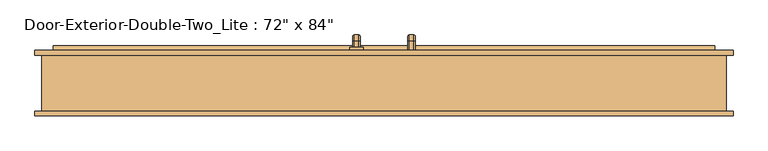
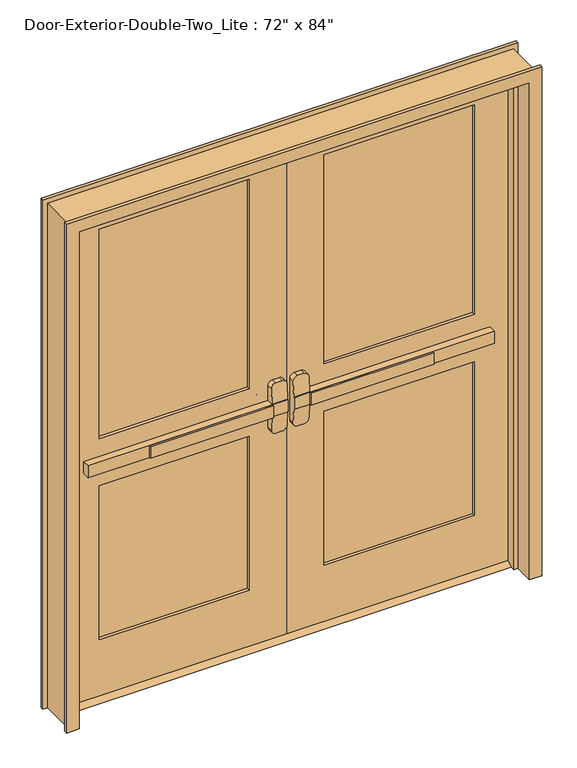
"""IFC4 building model written with IfcOpenShell, lengths in millimetres: door geometry."""

from ifc_helpers import new_model, si_unit, point, frame, frame_2d, origin, place, context, project, spatial, polyline, circle_curve, ellipse_curve, trimmed, segment, composite_curve, outline, extrude, faceted_brep, source, transform, mapped, element, save
from ifc_brep_helpers import plane_surface, cylinder_surface, revolved_surface, advanced_brep


def door_a6d348c0(model_context):
    return source(origin(), model_context, "Body", "SolidModel", [
        extrude(outline(polyline([(-575.7333333, 1.5875), (-575.7333333, 7.9375), (-76.2, 7.9375), (-76.2, 1.5875), (-575.7333333, 1.5875)])), frame((0.0, 0.0, 990.6), z_axis=(0.0, 0.0, 1.0), x_axis=(1.0, 0.0, 0.0)), (0.0, 0.0, 1.0), 50.8),
        advanced_brep(
        [(-12.7, 7.9375, 1041.4), (-76.2, 7.9375, 1041.4), (-825.5, 7.9375, 1041.4), (-825.5, 7.9375, 990.6), (-76.2, 7.9375, 990.6), (-12.7, 7.9375, 990.6), (-825.5, 39.6875, 1041.4), (-76.2, 39.6875, 1041.4), (-76.2, 39.6875, 1104.9), (-57.15, 39.6875, 1123.95), (-31.75, 39.6875, 1123.95), (-12.7, 39.6875, 1104.9), (-12.7, 39.6875, 927.1), (-31.75, 39.6875, 908.05), (-57.15, 39.6875, 908.05), (-76.2, 39.6875, 927.1), (-76.2, 39.6875, 990.6), (-825.5, 39.6875, 990.6), (-12.7, 11.1127467, 1041.4), (-76.2, 11.1127467, 1041.4), (-12.7, 11.1127467, 990.6), (-12.7, 16.1229269, 927.1), (-12.7, 16.1229269, 1104.9), (-76.2, 11.1127467, 990.6), (-76.2, 16.1229269, 1104.9), (-76.2, 16.1229269, 927.1), (-57.15, 17.625981, 1123.95), (-31.75, 17.625981, 1123.95), (-31.75, 17.625981, 908.05), (-57.15, 17.625981, 908.05)],
        [
            (0, 1),
            (1, 2),
            (2, 3),
            (3, 4),
            (4, 5),
            (5, 0),
            (6, 7),
            (7, 8),
            (8, 9, circle_curve(frame((-57.15, 39.6875, 1104.9), z_axis=(0.0, 1.0, 0.0), x_axis=(-1.0, 0.0, 0.0)), 19.05)),
            (9, 10),
            (10, 11, circle_curve(frame((-31.75, 39.6875, 1104.9), z_axis=(0.0, 1.0, 0.0), x_axis=(-1.0, 0.0, 0.0)), 19.05)),
            (11, 12),
            (12, 13, circle_curve(frame((-31.75, 39.6875, 927.1), z_axis=(0.0, 1.0, 0.0), x_axis=(-1.0, 0.0, 0.0)), 19.05)),
            (13, 14),
            (14, 15, circle_curve(frame((-57.15, 39.6875, 927.1), z_axis=(0.0, 1.0, 0.0), x_axis=(-1.0, 0.0, 0.0)), 19.05)),
            (15, 16),
            (16, 17),
            (17, 6),
            (0, 18),
            (18, 19),
            (19, 7),
            (6, 2),
            (5, 20),
            (20, 21),
            (21, 12),
            (11, 22),
            (22, 18),
            (16, 23),
            (23, 20),
            (3, 17),
            (19, 24),
            (24, 8),
            (15, 25),
            (25, 23),
            (9, 26),
            (26, 27),
            (27, 10),
            (13, 28),
            (28, 29),
            (29, 14),
            (29, 25, ellipse_curve(frame((-57.15, 16.1229269, 927.1), z_axis=(0.0, 0.9969018152893365, 0.07865602756830282), x_axis=(0.0, -0.07865602756830208, 0.9969018152893365)), 19.1092038, 19.05)),
            (24, 26, ellipse_curve(frame((-57.15, 16.1229269, 1104.9), z_axis=(0.0, 0.9969018152893376, -0.07865602756828934), x_axis=(0.0, -0.078656027568288, -0.9969018152893377)), 19.1092038, 19.05)),
            (27, 22, ellipse_curve(frame((-31.75, 16.1229269, 1104.9), z_axis=(0.0, 0.9969018152893376, -0.07865602756828934), x_axis=(0.0, -0.078656027568288, -0.9969018152893377)), 19.1092038, 19.05)),
            (21, 28, ellipse_curve(frame((-31.75, 16.1229269, 927.1), z_axis=(0.0, 0.9969018152893365, 0.07865602756830282), x_axis=(0.0, -0.07865602756830208, 0.9969018152893365)), 19.1092038, 19.05)),
        ],
        [
            plane_surface(frame((-12.7, 7.9375, 1041.4), z_axis=(0.0, -1.0, 0.0), x_axis=(1.0, 0.0, 0.0))),
            plane_surface(frame((-12.7, 39.6875, 1041.4), z_axis=(0.0, 1.0, 0.0), x_axis=(-1.0, 0.0, 0.0))),
            plane_surface(frame((-825.5, 7.9375, 1041.4), z_axis=(0.0, 0.0, 1.0), x_axis=(0.0, 1.0, 0.0))),
            plane_surface(frame((-12.7, 7.9375, 1041.4), z_axis=(1.0, 0.0, 0.0), x_axis=(0.0, 1.0, 0.0))),
            plane_surface(frame((-12.7, 7.9375, 990.6), z_axis=(0.0, 0.0, -1.0), x_axis=(0.0, 1.0, 0.0))),
            plane_surface(frame((-825.5, 7.9375, 990.6), z_axis=(-1.0, 0.0, 0.0), x_axis=(0.0, 1.0, 0.0))),
            plane_surface(frame((-76.2, 11.1127467, 927.1), z_axis=(-1.0, 0.0, 0.0), x_axis=(0.0, 1.0, 0.0))),
            plane_surface(frame((-57.15, 11.1127467, 1123.95), z_axis=(0.0, 0.0, 1.0), x_axis=(0.0, 1.0, 0.0))),
            plane_surface(frame((-31.75, 11.1127467, 908.05), z_axis=(0.0, 0.0, -1.0), x_axis=(0.0, 1.0, 0.0))),
            cylinder_surface(frame((-57.15, 39.6875, 927.1), z_axis=(0.0, -1.0, 0.0), x_axis=(-1.0, 0.0, 0.0)), 19.05),
            cylinder_surface(frame((-57.15, 39.6875, 1104.9), z_axis=(0.0, -1.0, 0.0), x_axis=(-1.0, 0.0, 0.0)), 19.05),
            cylinder_surface(frame((-31.75, 39.6875, 1104.9), z_axis=(0.0, -1.0, 0.0), x_axis=(-1.0, 0.0, 0.0)), 19.05),
            cylinder_surface(frame((-31.75, 39.6875, 927.1), z_axis=(0.0, -1.0, 0.0), x_axis=(-1.0, 0.0, 0.0)), 19.05),
            plane_surface(frame((-76.2, 11.1127467, 1041.4), z_axis=(0.0, -0.9969018152893376, 0.07865602756828934), x_axis=(1.0, 0.0, 0.0))),
            plane_surface(frame((-76.2, 17.625981, 908.05), z_axis=(0.0, -0.9969018152893365, -0.07865602756830282), x_axis=(1.0, 0.0, 0.0))),
        ],
        [
            (0, [[1, 2, 3, 4, 5, 6]]),
            (1, [[7, 8, 9, 10, 11, 12, 13, 14, 15, 16, 17, 18]]),
            (2, [[-2, -1, 19, 20, 21, -7, 22]]),
            (3, [[23, 24, 25, -12, 26, 27, -19, -6]]),
            (4, [[-17, 28, 29, -23, -5, -4, 30]]),
            (5, [[-22, -18, -30, -3]]),
            (6, [[-21, 31, 32, -8]]),
            (6, [[33, 34, -28, -16]]),
            (7, [[35, 36, 37, -10]]),
            (8, [[38, 39, 40, -14]]),
            (9, [[-40, 41, -33, -15]]),
            (10, [[-32, 42, -35, -9]]),
            (11, [[-37, 43, -26, -11]]),
            (12, [[-25, 44, -38, -13]]),
            (13, [[-27, -43, -36, -42, -31, -20]]),
            (14, [[-29, -34, -41, -39, -44, -24]]),
        ],
    ),
        extrude(outline(polyline([(84.1375, 12.7), (109.5375, 0.0), (14.2875, 0.0), (39.6875, 12.7), (84.1375, 12.7)])), frame((-914.4, 0.0, 0.0), z_axis=(1.0, 0.0, 0.0), x_axis=(0.0, 1.0, 0.0)), (0.0, 0.0, 1.0), 1828.8),
        extrude(outline(polyline([(575.7333333, 1.5875), (76.2, 1.5875), (76.2, 7.9375), (575.7333333, 7.9375), (575.7333333, 1.5875)])), frame((0.0, 0.0, 990.6), z_axis=(0.0, 0.0, 1.0), x_axis=(1.0, 0.0, 0.0)), (0.0, 0.0, 1.0), 50.8),
        advanced_brep(
        [(12.7, 7.9375, 1041.4), (12.7, 7.9375, 990.6), (76.2, 7.9375, 990.6), (825.5, 7.9375, 990.6), (825.5, 7.9375, 1041.4), (76.2, 7.9375, 1041.4), (825.5, 39.6875, 1041.4), (825.5, 39.6875, 990.6), (76.2, 39.6875, 990.6), (76.2, 39.6875, 927.1), (57.15, 39.6875, 908.05), (31.75, 39.6875, 908.05), (12.7, 39.6875, 927.1), (12.7, 39.6875, 1104.9), (31.75, 39.6875, 1123.95), (57.15, 39.6875, 1123.95), (76.2, 39.6875, 1104.9), (76.2, 39.6875, 1041.4), (76.2, 11.1127467, 1041.4), (12.7, 11.1127467, 1041.4), (12.7, 16.1229269, 1104.9), (12.7, 16.1229269, 927.1), (12.7, 11.1127467, 990.6), (76.2, 11.1127467, 990.6), (76.2, 16.1229269, 927.1), (76.2, 16.1229269, 1104.9), (31.75, 17.625981, 1123.95), (57.15, 17.625981, 1123.95), (57.15, 17.625981, 908.05), (31.75, 17.625981, 908.05)],
        [
            (0, 1),
            (1, 2),
            (2, 3),
            (3, 4),
            (4, 5),
            (5, 0),
            (6, 7),
            (7, 8),
            (8, 9),
            (9, 10, circle_curve(frame((57.15, 39.6875, 927.1), z_axis=(0.0, 1.0, 0.0), x_axis=(1.0, 0.0, 0.0)), 19.05)),
            (10, 11),
            (11, 12, circle_curve(frame((31.75, 39.6875, 927.1), z_axis=(0.0, 1.0, 0.0), x_axis=(1.0, 0.0, 0.0)), 19.05)),
            (12, 13),
            (13, 14, circle_curve(frame((31.75, 39.6875, 1104.9), z_axis=(0.0, 1.0, 0.0), x_axis=(1.0, 0.0, 0.0)), 19.05)),
            (14, 15),
            (15, 16, circle_curve(frame((57.15, 39.6875, 1104.9), z_axis=(0.0, 1.0, 0.0), x_axis=(1.0, 0.0, 0.0)), 19.05)),
            (16, 17),
            (17, 6),
            (4, 6),
            (17, 18),
            (18, 19),
            (19, 0),
            (19, 20),
            (20, 13),
            (12, 21),
            (21, 22),
            (22, 1),
            (7, 3),
            (22, 23),
            (23, 8),
            (23, 24),
            (24, 9),
            (16, 25),
            (25, 18),
            (14, 26),
            (26, 27),
            (27, 15),
            (10, 28),
            (28, 29),
            (29, 11),
            (24, 28, ellipse_curve(frame((57.15, 16.1229269, 927.1), z_axis=(0.0, 0.9969018152893365, 0.07865602756830282), x_axis=(0.0, -0.07865602756830208, 0.9969018152893365)), 19.1092038, 19.05)),
            (27, 25, ellipse_curve(frame((57.15, 16.1229269, 1104.9), z_axis=(0.0, 0.9969018152893376, -0.07865602756828934), x_axis=(0.0, -0.078656027568288, -0.9969018152893377)), 19.1092038, 19.05)),
            (20, 26, ellipse_curve(frame((31.75, 16.1229269, 1104.9), z_axis=(0.0, 0.9969018152893376, -0.07865602756828934), x_axis=(0.0, -0.078656027568288, -0.9969018152893377)), 19.1092038, 19.05)),
            (29, 21, ellipse_curve(frame((31.75, 16.1229269, 927.1), z_axis=(0.0, 0.9969018152893365, 0.07865602756830282), x_axis=(0.0, -0.07865602756830208, 0.9969018152893365)), 19.1092038, 19.05)),
        ],
        [
            plane_surface(frame((12.7, 7.9375, 1041.4), z_axis=(0.0, -1.0, 0.0), x_axis=(-1.0, 0.0, 0.0))),
            plane_surface(frame((12.7, 39.6875, 1041.4), z_axis=(0.0, 1.0, 0.0), x_axis=(1.0, 0.0, 0.0))),
            plane_surface(frame((825.5, 7.9375, 1041.4), z_axis=(0.0, 0.0, 1.0), x_axis=(0.0, 1.0, 0.0))),
            plane_surface(frame((12.7, 7.9375, 1041.4), z_axis=(-1.0, 0.0, 0.0), x_axis=(0.0, 1.0, 0.0))),
            plane_surface(frame((12.7, 7.9375, 990.6), z_axis=(0.0, 0.0, -1.0), x_axis=(0.0, 1.0, 0.0))),
            plane_surface(frame((825.5, 7.9375, 990.6), z_axis=(1.0, 0.0, 0.0), x_axis=(0.0, 1.0, 0.0))),
            plane_surface(frame((76.2, 11.1127467, 927.1), z_axis=(1.0, 0.0, 0.0), x_axis=(0.0, 1.0, 0.0))),
            plane_surface(frame((57.15, 11.1127467, 1123.95), z_axis=(0.0, 0.0, 1.0), x_axis=(0.0, 1.0, 0.0))),
            plane_surface(frame((31.75, 11.1127467, 908.05), z_axis=(0.0, 0.0, -1.0), x_axis=(0.0, 1.0, 0.0))),
            cylinder_surface(frame((57.15, 39.6875, 927.1), z_axis=(0.0, -1.0, 0.0), x_axis=(1.0, 0.0, 0.0)), 19.05),
            cylinder_surface(frame((57.15, 39.6875, 1104.9), z_axis=(0.0, -1.0, 0.0), x_axis=(1.0, 0.0, 0.0)), 19.05),
            cylinder_surface(frame((31.75, 39.6875, 1104.9), z_axis=(0.0, -1.0, 0.0), x_axis=(1.0, 0.0, 0.0)), 19.05),
            cylinder_surface(frame((31.75, 39.6875, 927.1), z_axis=(0.0, -1.0, 0.0), x_axis=(1.0, 0.0, 0.0)), 19.05),
            plane_surface(frame((76.2, 11.1127467, 1041.4), z_axis=(0.0, -0.9969018152893376, 0.07865602756828934), x_axis=(-1.0, 0.0, 0.0))),
            plane_surface(frame((76.2, 17.625981, 908.05), z_axis=(0.0, -0.9969018152893365, -0.07865602756830282), x_axis=(-1.0, 0.0, 0.0))),
        ],
        [
            (0, [[1, 2, 3, 4, 5, 6]]),
            (1, [[7, 8, 9, 10, 11, 12, 13, 14, 15, 16, 17, 18]]),
            (2, [[19, -18, 20, 21, 22, -6, -5]]),
            (3, [[-1, -22, 23, 24, -13, 25, 26, 27]]),
            (4, [[28, -3, -2, -27, 29, 30, -8]]),
            (5, [[-4, -28, -7, -19]]),
            (6, [[-9, -30, 31, 32]]),
            (6, [[-17, 33, 34, -20]]),
            (7, [[-15, 35, 36, 37]]),
            (8, [[-11, 38, 39, 40]]),
            (9, [[-10, -32, 41, -38]]),
            (10, [[-16, -37, 42, -33]]),
            (11, [[-14, -24, 43, -35]]),
            (12, [[-12, -40, 44, -25]]),
            (13, [[-21, -34, -42, -36, -43, -23]]),
            (14, [[-26, -44, -39, -41, -31, -29]]),
        ],
    ),
        advanced_brep(
        [(66.2, 96.8375, 1017.190625), (66.2, 96.8375, 1014.809375), (69.771875, 96.8375, 1011.2375), (82.6284594, 96.8375, 1011.2375), (86.2, 96.8375, 1014.8090406), (86.2, 96.8375, 1017.190625), (82.628125, 96.8375, 1020.7625), (69.771875, 96.8375, 1020.7625), (66.2, 96.8375, 887.809375), (69.771875, 96.8375, 884.2375), (82.628125, 96.8375, 884.2375), (86.2, 96.8375, 887.809375), (86.2, 96.8375, 890.1909594), (82.6284594, 96.8375, 893.7625), (69.771875, 96.8375, 893.7625), (66.2, 96.8375, 890.190625), (66.2, 122.2375, 1017.190625), (66.2, 136.128125, 1003.3), (66.2, 136.128125, 901.7), (66.2, 122.2375, 887.809375), (66.2, 122.2375, 890.190625), (66.2, 133.746875, 901.7), (66.2, 133.746875, 1003.3), (66.2, 122.2375, 1014.809375), (69.771875, 122.2375, 1011.2375), (82.6284594, 122.2375, 1011.2375), (86.2, 122.2375, 1014.8090406), (86.2, 133.7465406, 1003.3), (86.2, 133.7465406, 901.7), (86.2, 122.2375, 890.1909594), (86.2, 122.2375, 887.809375), (86.2, 136.128125, 901.7), (86.2, 136.128125, 1003.3), (86.2, 122.2375, 1017.190625), (82.628125, 122.2375, 1020.7625), (69.771875, 122.2375, 1020.7625), (69.771875, 130.175, 1003.3), (82.6284594, 130.175, 1003.3), (82.628125, 139.7, 1003.3), (69.771875, 139.7, 1003.3), (69.771875, 130.175, 901.7), (82.6284594, 130.175, 901.7), (82.628125, 139.7, 901.7), (69.771875, 139.7, 901.7), (69.771875, 122.2375, 893.7625), (82.6284594, 122.2375, 893.7625), (82.628125, 122.2375, 884.2375), (69.771875, 122.2375, 884.2375)],
        [
            (0, 1),
            (1, 2, circle_curve(frame((69.771875, 96.8375, 1014.809375), z_axis=(0.0, -1.0, 0.0), x_axis=(0.0, 0.0, 1.0)), 3.571875)),
            (2, 3),
            (3, 4, circle_curve(frame((82.6284594, 96.8375, 1014.8090406), z_axis=(0.0, -1.0, 0.0), x_axis=(0.0, 0.0, 1.0)), 3.5715406)),
            (4, 5),
            (5, 6, circle_curve(frame((82.628125, 96.8375, 1017.190625), z_axis=(0.0, -1.0, 0.0), x_axis=(0.0, 0.0, 1.0)), 3.571875)),
            (6, 7),
            (7, 0, circle_curve(frame((69.771875, 96.8375, 1017.190625), z_axis=(0.0, -1.0, 0.0), x_axis=(0.0, 0.0, 1.0)), 3.571875)),
            (8, 9, circle_curve(frame((69.771875, 96.8375, 887.809375), z_axis=(0.0, -1.0, 0.0), x_axis=(0.0, 0.0, -1.0)), 3.571875)),
            (9, 10),
            (10, 11, circle_curve(frame((82.628125, 96.8375, 887.809375), z_axis=(0.0, -1.0, 0.0), x_axis=(0.0, 0.0, -1.0)), 3.571875)),
            (11, 12),
            (12, 13, circle_curve(frame((82.6284594, 96.8375, 890.1909594), z_axis=(0.0, -1.0, 0.0), x_axis=(0.0, 0.0, -1.0)), 3.5715406)),
            (13, 14),
            (14, 15, circle_curve(frame((69.771875, 96.8375, 890.190625), z_axis=(0.0, -1.0, 0.0), x_axis=(0.0, 0.0, -1.0)), 3.571875)),
            (15, 8),
            (0, 16),
            (16, 17, circle_curve(frame((66.2, 122.2375, 1003.3), z_axis=(-1.0, 0.0, 0.0), x_axis=(0.0, 0.0, 1.0)), 13.890625)),
            (17, 18),
            (18, 19, circle_curve(frame((66.2, 122.2375, 901.7), z_axis=(-1.0, 0.0, 0.0), x_axis=(0.0, 1.0, 0.0)), 13.890625)),
            (19, 8),
            (15, 20),
            (20, 21, circle_curve(frame((66.2, 122.2375, 901.7), z_axis=(1.0, 0.0, 0.0), x_axis=(0.0, 1.0, 0.0)), 11.509375)),
            (21, 22),
            (22, 23, circle_curve(frame((66.2, 122.2375, 1003.3), z_axis=(1.0, 0.0, 0.0), x_axis=(0.0, 0.0, 1.0)), 11.509375)),
            (23, 1),
            (23, 24, circle_curve(frame((69.771875, 122.2375, 1014.809375), z_axis=(0.0, -1.0, 0.0), x_axis=(0.0, 0.0, 1.0)), 3.571875)),
            (24, 2),
            (24, 25),
            (25, 3),
            (25, 26, circle_curve(frame((82.6284594, 122.2375, 1014.8090406), z_axis=(0.0, -1.0, 0.0), x_axis=(0.0, 0.0, 1.0)), 3.5715406)),
            (26, 4),
            (26, 27, circle_curve(frame((86.2, 122.2375, 1003.3), z_axis=(-1.0, 0.0, 0.0), x_axis=(0.0, 0.0, 1.0)), 11.5090406)),
            (27, 28),
            (28, 29, circle_curve(frame((86.2, 122.2375, 901.7), z_axis=(-1.0, 0.0, 0.0), x_axis=(0.0, 1.0, 0.0)), 11.5090406)),
            (29, 12),
            (11, 30),
            (30, 31, circle_curve(frame((86.2, 122.2375, 901.7), z_axis=(1.0, 0.0, 0.0), x_axis=(0.0, 1.0, 0.0)), 13.890625)),
            (31, 32),
            (32, 33, circle_curve(frame((86.2, 122.2375, 1003.3), z_axis=(1.0, 0.0, 0.0), x_axis=(0.0, 0.0, 1.0)), 13.890625)),
            (33, 5),
            (33, 34, circle_curve(frame((82.628125, 122.2375, 1017.190625), z_axis=(0.0, -1.0, 0.0), x_axis=(0.0, 0.0, 1.0)), 3.571875)),
            (34, 6),
            (34, 35),
            (35, 7),
            (35, 16, circle_curve(frame((69.771875, 122.2375, 1017.190625), z_axis=(0.0, -1.0, 0.0), x_axis=(0.0, 0.0, 1.0)), 3.571875)),
            (36, 24, circle_curve(frame((69.771875, 122.2375, 1003.3), z_axis=(1.0, 0.0, 0.0), x_axis=(0.0, 0.0, 1.0)), 7.9375)),
            (22, 36, circle_curve(frame((69.771875, 133.746875, 1003.3), z_axis=(0.0, 0.0, 1.0), x_axis=(0.0, 1.0, 0.0)), 3.571875)),
            (37, 25, circle_curve(frame((82.6284594, 122.2375, 1003.3), z_axis=(1.0, 0.0, 0.0), x_axis=(0.0, 0.0, 1.0)), 7.9375)),
            (36, 37),
            (37, 27, circle_curve(frame((82.6284594, 133.7465406, 1003.3), z_axis=(0.0, 0.0, 1.0), x_axis=(0.0, 1.0, 0.0)), 3.5715406)),
            (38, 34, circle_curve(frame((82.628125, 122.2375, 1003.3), z_axis=(1.0, 0.0, 0.0), x_axis=(0.0, 0.0, 1.0)), 17.4625)),
            (32, 38, circle_curve(frame((82.628125, 136.128125, 1003.3), z_axis=(0.0, 0.0, 1.0), x_axis=(0.0, 1.0, 0.0)), 3.571875)),
            (39, 35, circle_curve(frame((69.771875, 122.2375, 1003.3), z_axis=(1.0, 0.0, 0.0), x_axis=(0.0, 0.0, 1.0)), 17.4625)),
            (38, 39),
            (39, 17, circle_curve(frame((69.771875, 136.128125, 1003.3), z_axis=(0.0, 0.0, 1.0), x_axis=(0.0, 1.0, 0.0)), 3.571875)),
            (21, 40, circle_curve(frame((69.771875, 133.746875, 901.7), z_axis=(0.0, 0.0, 1.0), x_axis=(0.0, 1.0, 0.0)), 3.571875)),
            (40, 36),
            (40, 41),
            (41, 37),
            (41, 28, circle_curve(frame((82.6284594, 133.7465406, 901.7), z_axis=(0.0, 0.0, 1.0), x_axis=(0.0, 1.0, 0.0)), 3.5715406)),
            (31, 42, circle_curve(frame((82.628125, 136.128125, 901.7), z_axis=(0.0, 0.0, 1.0), x_axis=(0.0, 1.0, 0.0)), 3.571875)),
            (42, 38),
            (42, 43),
            (43, 39),
            (43, 18, circle_curve(frame((69.771875, 136.128125, 901.7), z_axis=(0.0, 0.0, 1.0), x_axis=(0.0, 1.0, 0.0)), 3.571875)),
            (44, 40, circle_curve(frame((69.771875, 122.2375, 901.7), z_axis=(1.0, 0.0, 0.0), x_axis=(0.0, 1.0, 0.0)), 7.9375)),
            (20, 44, circle_curve(frame((69.771875, 122.2375, 890.190625), z_axis=(0.0, 1.0, 0.0), x_axis=(0.0, 0.0, -1.0)), 3.571875)),
            (45, 41, circle_curve(frame((82.6284594, 122.2375, 901.7), z_axis=(1.0, 0.0, 0.0), x_axis=(0.0, 1.0, 0.0)), 7.9375)),
            (44, 45),
            (45, 29, circle_curve(frame((82.6284594, 122.2375, 890.1909594), z_axis=(0.0, 1.0, 0.0), x_axis=(0.0, 0.0, -1.0)), 3.5715406)),
            (46, 42, circle_curve(frame((82.628125, 122.2375, 901.7), z_axis=(1.0, 0.0, 0.0), x_axis=(0.0, 1.0, 0.0)), 17.4625)),
            (30, 46, circle_curve(frame((82.628125, 122.2375, 887.809375), z_axis=(0.0, 1.0, 0.0), x_axis=(0.0, 0.0, -1.0)), 3.571875)),
            (47, 43, circle_curve(frame((69.771875, 122.2375, 901.7), z_axis=(1.0, 0.0, 0.0), x_axis=(0.0, 1.0, 0.0)), 17.4625)),
            (46, 47),
            (47, 19, circle_curve(frame((69.771875, 122.2375, 887.809375), z_axis=(0.0, 1.0, 0.0), x_axis=(0.0, 0.0, -1.0)), 3.571875)),
            (14, 44),
            (13, 45),
            (10, 46),
            (9, 47),
        ],
        [
            plane_surface(frame((76.2, 96.8375, 1016.0), z_axis=(0.0, -1.0, 0.0), x_axis=(1.0, 0.0, 0.0))),
            plane_surface(frame((76.2, 96.8375, 889.0), z_axis=(0.0, -1.0, 0.0), x_axis=(1.0, 0.0, 0.0))),
            plane_surface(frame((66.2, 96.8375, 1017.190625), z_axis=(-1.0, 0.0, 0.0), x_axis=(0.0, 1.0, 0.0))),
            cylinder_surface(frame((69.771875, 96.8375, 1014.809375), z_axis=(0.0, -1.0, 0.0), x_axis=(0.0, 0.0, 1.0)), 3.571875),
            plane_surface(frame((69.771875, 96.8375, 1011.2375), z_axis=(0.0, 0.0, -1.0), x_axis=(0.0, 1.0, 0.0))),
            cylinder_surface(frame((82.6284594, 96.8375, 1014.8090406), z_axis=(0.0, -1.0, 0.0), x_axis=(0.0, 0.0, 1.0)), 3.5715406),
            plane_surface(frame((86.2, 96.8375, 1014.8090406), z_axis=(1.0, 0.0, 0.0), x_axis=(0.0, 1.0, 0.0))),
            cylinder_surface(frame((82.628125, 96.8375, 1017.190625), z_axis=(0.0, -1.0, 0.0), x_axis=(0.0, 0.0, 1.0)), 3.571875),
            plane_surface(frame((82.628125, 96.8375, 1020.7625), z_axis=(0.0, 0.0, 1.0), x_axis=(0.0, 1.0, 0.0))),
            cylinder_surface(frame((69.771875, 96.8375, 1017.190625), z_axis=(0.0, -1.0, 0.0), x_axis=(0.0, 0.0, 1.0)), 3.571875),
            revolved_surface(trimmed(ellipse_curve(frame((69.771875, 122.2375, 1014.809375), z_axis=(0.0, -1.0, 0.0), x_axis=(0.0, 0.0, 1.0)), 3.571875, 3.571875), [point((66.2, 122.2375, 1014.809375))], [point((69.771875, 122.2375, 1011.2375))], True, "CARTESIAN"), (76.2, 122.2375, 1003.3), (-1.0, 0.0, 0.0)),
            revolved_surface(polyline([(69.771875, 122.2375, 1011.2375), (82.6284594, 122.2375, 1011.2375)]), (76.2, 122.2375, 1003.3), (-1.0, 0.0, 0.0)),
            revolved_surface(trimmed(ellipse_curve(frame((82.6284594, 122.2375, 1014.8090406), z_axis=(0.0, -1.0, 0.0), x_axis=(0.0, 0.0, 1.0)), 3.5715406, 3.5715406), [point((82.6284594, 122.2375, 1011.2375))], [point((86.2, 122.2375, 1014.8090406))], True, "CARTESIAN"), (76.2, 122.2375, 1003.3), (-1.0, 0.0, 0.0)),
            revolved_surface(trimmed(ellipse_curve(frame((82.628125, 122.2375, 1017.190625), z_axis=(0.0, -1.0, 0.0), x_axis=(0.0, 0.0, 1.0)), 3.571875, 3.571875), [point((86.2, 122.2375, 1017.190625))], [point((82.628125, 122.2375, 1020.7625))], True, "CARTESIAN"), (76.2, 122.2375, 1003.3), (-1.0, 0.0, 0.0)),
            cylinder_surface(frame((76.2, 122.2375, 1003.3), z_axis=(-1.0, 0.0, 0.0), x_axis=(0.0, 0.0, 1.0)), 17.4625),
            revolved_surface(trimmed(ellipse_curve(frame((69.771875, 122.2375, 1017.190625), z_axis=(0.0, -1.0, 0.0), x_axis=(0.0, 0.0, 1.0)), 3.571875, 3.571875), [point((69.771875, 122.2375, 1020.7625))], [point((66.2, 122.2375, 1017.190625))], True, "CARTESIAN"), (76.2, 122.2375, 1003.3), (-1.0, 0.0, 0.0)),
            cylinder_surface(frame((69.771875, 133.746875, 1003.3), z_axis=(0.0, 0.0, 1.0), x_axis=(0.0, 1.0, 0.0)), 3.571875),
            plane_surface(frame((69.771875, 130.175, 1003.3), z_axis=(0.0, -1.0, 0.0), x_axis=(0.0, 0.0, -1.0))),
            cylinder_surface(frame((82.6284594, 133.7465406, 1003.3), z_axis=(0.0, 0.0, 1.0), x_axis=(0.0, 1.0, 0.0)), 3.5715406),
            cylinder_surface(frame((82.628125, 136.128125, 1003.3), z_axis=(0.0, 0.0, 1.0), x_axis=(0.0, 1.0, 0.0)), 3.571875),
            plane_surface(frame((82.628125, 139.7, 1003.3), z_axis=(0.0, 1.0, 0.0), x_axis=(0.0, 0.0, -1.0))),
            cylinder_surface(frame((69.771875, 136.128125, 1003.3), z_axis=(0.0, 0.0, 1.0), x_axis=(0.0, 1.0, 0.0)), 3.571875),
            revolved_surface(trimmed(ellipse_curve(frame((69.771875, 133.746875, 901.7), z_axis=(0.0, 0.0, 1.0), x_axis=(0.0, 1.0, 0.0)), 3.571875, 3.571875), [point((66.2, 133.746875, 901.7))], [point((69.771875, 130.175, 901.7))], True, "CARTESIAN"), (76.2, 122.2375, 901.7), (-1.0, 0.0, 0.0)),
            revolved_surface(polyline([(69.771875, 130.175, 901.7), (82.6284594, 130.175, 901.7)]), (76.2, 122.2375, 901.7), (-1.0, 0.0, 0.0)),
            revolved_surface(trimmed(ellipse_curve(frame((82.6284594, 133.7465406, 901.7), z_axis=(0.0, 0.0, 1.0), x_axis=(0.0, 1.0, 0.0)), 3.5715406, 3.5715406), [point((82.6284594, 130.175, 901.7))], [point((86.2, 133.7465406, 901.7))], True, "CARTESIAN"), (76.2, 122.2375, 901.7), (-1.0, 0.0, 0.0)),
            revolved_surface(trimmed(ellipse_curve(frame((82.628125, 136.128125, 901.7), z_axis=(0.0, 0.0, 1.0), x_axis=(0.0, 1.0, 0.0)), 3.571875, 3.571875), [point((86.2, 136.128125, 901.7))], [point((82.628125, 139.7, 901.7))], True, "CARTESIAN"), (76.2, 122.2375, 901.7), (-1.0, 0.0, 0.0)),
            cylinder_surface(frame((76.2, 122.2375, 901.7), z_axis=(-1.0, 0.0, 0.0), x_axis=(0.0, 1.0, 0.0)), 17.4625),
            revolved_surface(trimmed(ellipse_curve(frame((69.771875, 136.128125, 901.7), z_axis=(0.0, 0.0, 1.0), x_axis=(0.0, 1.0, 0.0)), 3.571875, 3.571875), [point((69.771875, 139.7, 901.7))], [point((66.2, 136.128125, 901.7))], True, "CARTESIAN"), (76.2, 122.2375, 901.7), (-1.0, 0.0, 0.0)),
            cylinder_surface(frame((69.771875, 122.2375, 890.190625), z_axis=(0.0, 1.0, 0.0), x_axis=(0.0, 0.0, -1.0)), 3.571875),
            plane_surface(frame((69.771875, 122.2375, 893.7625), z_axis=(0.0, 0.0, 1.0), x_axis=(0.0, -1.0, 0.0))),
            cylinder_surface(frame((82.6284594, 122.2375, 890.1909594), z_axis=(0.0, 1.0, 0.0), x_axis=(0.0, 0.0, -1.0)), 3.5715406),
            cylinder_surface(frame((82.628125, 122.2375, 887.809375), z_axis=(0.0, 1.0, 0.0), x_axis=(0.0, 0.0, -1.0)), 3.571875),
            plane_surface(frame((82.628125, 122.2375, 884.2375), z_axis=(0.0, 0.0, -1.0), x_axis=(0.0, -1.0, 0.0))),
            cylinder_surface(frame((69.771875, 122.2375, 887.809375), z_axis=(0.0, 1.0, 0.0), x_axis=(0.0, 0.0, -1.0)), 3.571875),
        ],
        [
            (0, [[1, 2, 3, 4, 5, 6, 7, 8]]),
            (1, [[9, 10, 11, 12, 13, 14, 15, 16]]),
            (2, [[-1, 17, 18, 19, 20, 21, -16, 22, 23, 24, 25, 26]]),
            (3, [[-2, -26, 27, 28]]),
            (4, [[-3, -28, 29, 30]]),
            (5, [[-4, -30, 31, 32]]),
            (6, [[-5, -32, 33, 34, 35, 36, -12, 37, 38, 39, 40, 41]]),
            (7, [[-6, -41, 42, 43]]),
            (8, [[-7, -43, 44, 45]]),
            (9, [[-8, -45, 46, -17]]),
            (10, [[47, -27, -25, 48]]),
            (11, [[49, -29, -47, 50]]),
            (12, [[-33, -31, -49, 51]]),
            (13, [[52, -42, -40, 53]]),
            (14, [[54, -44, -52, 55]]),
            (15, [[-18, -46, -54, 56]]),
            (16, [[-48, -24, 57, 58]]),
            (17, [[-50, -58, 59, 60]]),
            (18, [[-51, -60, 61, -34]]),
            (19, [[-53, -39, 62, 63]]),
            (20, [[-55, -63, 64, 65]]),
            (21, [[-56, -65, 66, -19]]),
            (22, [[67, -57, -23, 68]]),
            (23, [[69, -59, -67, 70]]),
            (24, [[-35, -61, -69, 71]]),
            (25, [[72, -62, -38, 73]]),
            (26, [[74, -64, -72, 75]]),
            (27, [[-20, -66, -74, 76]]),
            (28, [[-68, -22, -15, 77]]),
            (29, [[-70, -77, -14, 78]]),
            (30, [[-71, -78, -13, -36]]),
            (31, [[-73, -37, -11, 79]]),
            (32, [[-75, -79, -10, 80]]),
            (33, [[-76, -80, -9, -21]]),
        ],
    ),
        extrude(outline(composite_curve([segment(trimmed(circle_curve(frame_2d((1113.0338574, 76.2)), 89.3016225), [point((1193.8, 114.3))], [point((1193.8, 38.1))], False, "CARTESIAN"), True, "CONTINUOUS"), segment(polyline([(1193.8, 38.1), (838.2, 38.1)]), True, "CONTINUOUS"), segment(trimmed(circle_curve(frame_2d((918.9661426, 76.2)), 89.3016225), [point((838.2, 38.1))], [point((838.2, 114.3))], False, "CARTESIAN"), True, "CONTINUOUS"), segment(polyline([(838.2, 114.3), (1193.8, 114.3)]), True, "CONTINUOUS")], self_intersect=False)), frame((0.0, 84.1375, 0.0), z_axis=(0.0, 1.0, 0.0), x_axis=(0.0, 0.0, 1.0)), (0.0, 0.0, 1.0), 12.7),
        advanced_brep(
        [(-86.2, 96.8375, 1017.190625), (-86.2, 96.8375, 1014.809375), (-82.628125, 96.8375, 1011.2375), (-69.7715406, 96.8375, 1011.2375), (-66.2, 96.8375, 1014.8090406), (-66.2, 96.8375, 1017.190625), (-69.771875, 96.8375, 1020.7625), (-82.628125, 96.8375, 1020.7625), (-86.2, 96.8375, 887.809375), (-82.628125, 96.8375, 884.2375), (-69.771875, 96.8375, 884.2375), (-66.2, 96.8375, 887.809375), (-66.2, 96.8375, 890.1909594), (-69.7715406, 96.8375, 893.7625), (-82.628125, 96.8375, 893.7625), (-86.2, 96.8375, 890.190625), (-86.2, 122.2375, 1017.190625), (-86.2, 136.128125, 1003.3), (-86.2, 136.128125, 901.7), (-86.2, 122.2375, 887.809375), (-86.2, 122.2375, 890.190625), (-86.2, 133.746875, 901.7), (-86.2, 133.746875, 1003.3), (-86.2, 122.2375, 1014.809375), (-82.628125, 122.2375, 1011.2375), (-69.7715406, 122.2375, 1011.2375), (-66.2, 122.2375, 1014.8090406), (-66.2, 133.7465406, 1003.3), (-66.2, 133.7465406, 901.7), (-66.2, 122.2375, 890.1909594), (-66.2, 122.2375, 887.809375), (-66.2, 136.128125, 901.7), (-66.2, 136.128125, 1003.3), (-66.2, 122.2375, 1017.190625), (-69.771875, 122.2375, 1020.7625), (-82.628125, 122.2375, 1020.7625), (-82.628125, 130.175, 1003.3), (-69.7715406, 130.175, 1003.3), (-69.771875, 139.7, 1003.3), (-82.628125, 139.7, 1003.3), (-82.628125, 130.175, 901.7), (-69.7715406, 130.175, 901.7), (-69.771875, 139.7, 901.7), (-82.628125, 139.7, 901.7), (-82.628125, 122.2375, 893.7625), (-69.7715406, 122.2375, 893.7625), (-69.771875, 122.2375, 884.2375), (-82.628125, 122.2375, 884.2375)],
        [
            (0, 1),
            (1, 2, circle_curve(frame((-82.628125, 96.8375, 1014.809375), z_axis=(0.0, -1.0, 0.0), x_axis=(0.0, 0.0, 1.0)), 3.571875)),
            (2, 3),
            (3, 4, circle_curve(frame((-69.7715406, 96.8375, 1014.8090406), z_axis=(0.0, -1.0, 0.0), x_axis=(0.0, 0.0, 1.0)), 3.5715406)),
            (4, 5),
            (5, 6, circle_curve(frame((-69.771875, 96.8375, 1017.190625), z_axis=(0.0, -1.0, 0.0), x_axis=(0.0, 0.0, 1.0)), 3.571875)),
            (6, 7),
            (7, 0, circle_curve(frame((-82.628125, 96.8375, 1017.190625), z_axis=(0.0, -1.0, 0.0), x_axis=(0.0, 0.0, 1.0)), 3.571875)),
            (8, 9, circle_curve(frame((-82.628125, 96.8375, 887.809375), z_axis=(0.0, -1.0, 0.0), x_axis=(0.0, 0.0, -1.0)), 3.571875)),
            (9, 10),
            (10, 11, circle_curve(frame((-69.771875, 96.8375, 887.809375), z_axis=(0.0, -1.0, 0.0), x_axis=(0.0, 0.0, -1.0)), 3.571875)),
            (11, 12),
            (12, 13, circle_curve(frame((-69.7715406, 96.8375, 890.1909594), z_axis=(0.0, -1.0, 0.0), x_axis=(0.0, 0.0, -1.0)), 3.5715406)),
            (13, 14),
            (14, 15, circle_curve(frame((-82.628125, 96.8375, 890.190625), z_axis=(0.0, -1.0, 0.0), x_axis=(0.0, 0.0, -1.0)), 3.571875)),
            (15, 8),
            (0, 16),
            (16, 17, circle_curve(frame((-86.2, 122.2375, 1003.3), z_axis=(-1.0, 0.0, 0.0), x_axis=(0.0, 0.0, 1.0)), 13.890625)),
            (17, 18),
            (18, 19, circle_curve(frame((-86.2, 122.2375, 901.7), z_axis=(-1.0, 0.0, 0.0), x_axis=(0.0, 1.0, 0.0)), 13.890625)),
            (19, 8),
            (15, 20),
            (20, 21, circle_curve(frame((-86.2, 122.2375, 901.7), z_axis=(1.0, 0.0, 0.0), x_axis=(0.0, 1.0, 0.0)), 11.509375)),
            (21, 22),
            (22, 23, circle_curve(frame((-86.2, 122.2375, 1003.3), z_axis=(1.0, 0.0, 0.0), x_axis=(0.0, 0.0, 1.0)), 11.509375)),
            (23, 1),
            (23, 24, circle_curve(frame((-82.628125, 122.2375, 1014.809375), z_axis=(0.0, -1.0, 0.0), x_axis=(0.0, 0.0, 1.0)), 3.571875)),
            (24, 2),
            (24, 25),
            (25, 3),
            (25, 26, circle_curve(frame((-69.7715406, 122.2375, 1014.8090406), z_axis=(0.0, -1.0, 0.0), x_axis=(0.0, 0.0, 1.0)), 3.5715406)),
            (26, 4),
            (26, 27, circle_curve(frame((-66.2, 122.2375, 1003.3), z_axis=(-1.0, 0.0, 0.0), x_axis=(0.0, 0.0, 1.0)), 11.5090406)),
            (27, 28),
            (28, 29, circle_curve(frame((-66.2, 122.2375, 901.7), z_axis=(-1.0, 0.0, 0.0), x_axis=(0.0, 1.0, 0.0)), 11.5090406)),
            (29, 12),
            (11, 30),
            (30, 31, circle_curve(frame((-66.2, 122.2375, 901.7), z_axis=(1.0, 0.0, 0.0), x_axis=(0.0, 1.0, 0.0)), 13.890625)),
            (31, 32),
            (32, 33, circle_curve(frame((-66.2, 122.2375, 1003.3), z_axis=(1.0, 0.0, 0.0), x_axis=(0.0, 0.0, 1.0)), 13.890625)),
            (33, 5),
            (33, 34, circle_curve(frame((-69.771875, 122.2375, 1017.190625), z_axis=(0.0, -1.0, 0.0), x_axis=(0.0, 0.0, 1.0)), 3.571875)),
            (34, 6),
            (34, 35),
            (35, 7),
            (35, 16, circle_curve(frame((-82.628125, 122.2375, 1017.190625), z_axis=(0.0, -1.0, 0.0), x_axis=(0.0, 0.0, 1.0)), 3.571875)),
            (36, 24, circle_curve(frame((-82.628125, 122.2375, 1003.3), z_axis=(1.0, 0.0, 0.0), x_axis=(0.0, 0.0, 1.0)), 7.9375)),
            (22, 36, circle_curve(frame((-82.628125, 133.746875, 1003.3), z_axis=(0.0, 0.0, 1.0), x_axis=(0.0, 1.0, 0.0)), 3.571875)),
            (37, 25, circle_curve(frame((-69.7715406, 122.2375, 1003.3), z_axis=(1.0, 0.0, 0.0), x_axis=(0.0, 0.0, 1.0)), 7.9375)),
            (36, 37),
            (37, 27, circle_curve(frame((-69.7715406, 133.7465406, 1003.3), z_axis=(0.0, 0.0, 1.0), x_axis=(0.0, 1.0, 0.0)), 3.5715406)),
            (38, 34, circle_curve(frame((-69.771875, 122.2375, 1003.3), z_axis=(1.0, 0.0, 0.0), x_axis=(0.0, 0.0, 1.0)), 17.4625)),
            (32, 38, circle_curve(frame((-69.771875, 136.128125, 1003.3), z_axis=(0.0, 0.0, 1.0), x_axis=(0.0, 1.0, 0.0)), 3.571875)),
            (39, 35, circle_curve(frame((-82.628125, 122.2375, 1003.3), z_axis=(1.0, 0.0, 0.0), x_axis=(0.0, 0.0, 1.0)), 17.4625)),
            (38, 39),
            (39, 17, circle_curve(frame((-82.628125, 136.128125, 1003.3), z_axis=(0.0, 0.0, 1.0), x_axis=(0.0, 1.0, 0.0)), 3.571875)),
            (21, 40, circle_curve(frame((-82.628125, 133.746875, 901.7), z_axis=(0.0, 0.0, 1.0), x_axis=(0.0, 1.0, 0.0)), 3.571875)),
            (40, 36),
            (40, 41),
            (41, 37),
            (41, 28, circle_curve(frame((-69.7715406, 133.7465406, 901.7), z_axis=(0.0, 0.0, 1.0), x_axis=(0.0, 1.0, 0.0)), 3.5715406)),
            (31, 42, circle_curve(frame((-69.771875, 136.128125, 901.7), z_axis=(0.0, 0.0, 1.0), x_axis=(0.0, 1.0, 0.0)), 3.571875)),
            (42, 38),
            (42, 43),
            (43, 39),
            (43, 18, circle_curve(frame((-82.628125, 136.128125, 901.7), z_axis=(0.0, 0.0, 1.0), x_axis=(0.0, 1.0, 0.0)), 3.571875)),
            (44, 40, circle_curve(frame((-82.628125, 122.2375, 901.7), z_axis=(1.0, 0.0, 0.0), x_axis=(0.0, 1.0, 0.0)), 7.9375)),
            (20, 44, circle_curve(frame((-82.628125, 122.2375, 890.190625), z_axis=(0.0, 1.0, 0.0), x_axis=(0.0, 0.0, -1.0)), 3.571875)),
            (45, 41, circle_curve(frame((-69.7715406, 122.2375, 901.7), z_axis=(1.0, 0.0, 0.0), x_axis=(0.0, 1.0, 0.0)), 7.9375)),
            (44, 45),
            (45, 29, circle_curve(frame((-69.7715406, 122.2375, 890.1909594), z_axis=(0.0, 1.0, 0.0), x_axis=(0.0, 0.0, -1.0)), 3.5715406)),
            (46, 42, circle_curve(frame((-69.771875, 122.2375, 901.7), z_axis=(1.0, 0.0, 0.0), x_axis=(0.0, 1.0, 0.0)), 17.4625)),
            (30, 46, circle_curve(frame((-69.771875, 122.2375, 887.809375), z_axis=(0.0, 1.0, 0.0), x_axis=(0.0, 0.0, -1.0)), 3.571875)),
            (47, 43, circle_curve(frame((-82.628125, 122.2375, 901.7), z_axis=(1.0, 0.0, 0.0), x_axis=(0.0, 1.0, 0.0)), 17.4625)),
            (46, 47),
            (47, 19, circle_curve(frame((-82.628125, 122.2375, 887.809375), z_axis=(0.0, 1.0, 0.0), x_axis=(0.0, 0.0, -1.0)), 3.571875)),
            (14, 44),
            (13, 45),
            (10, 46),
            (9, 47),
        ],
        [
            plane_surface(frame((-76.2, 96.8375, 1016.0), z_axis=(0.0, -1.0, 0.0), x_axis=(1.0, 0.0, 0.0))),
            plane_surface(frame((-76.2, 96.8375, 889.0), z_axis=(0.0, -1.0, 0.0), x_axis=(1.0, 0.0, 0.0))),
            plane_surface(frame((-86.2, 96.8375, 1017.190625), z_axis=(-1.0, 0.0, 0.0), x_axis=(0.0, 1.0, 0.0))),
            cylinder_surface(frame((-82.628125, 96.8375, 1014.809375), z_axis=(0.0, -1.0, 0.0), x_axis=(0.0, 0.0, 1.0)), 3.571875),
            plane_surface(frame((-82.628125, 96.8375, 1011.2375), z_axis=(0.0, 0.0, -1.0), x_axis=(0.0, 1.0, 0.0))),
            cylinder_surface(frame((-69.7715406, 96.8375, 1014.8090406), z_axis=(0.0, -1.0, 0.0), x_axis=(0.0, 0.0, 1.0)), 3.5715406),
            plane_surface(frame((-66.2, 96.8375, 1014.8090406), z_axis=(1.0, 0.0, 0.0), x_axis=(0.0, 1.0, 0.0))),
            cylinder_surface(frame((-69.771875, 96.8375, 1017.190625), z_axis=(0.0, -1.0, 0.0), x_axis=(0.0, 0.0, 1.0)), 3.571875),
            plane_surface(frame((-69.771875, 96.8375, 1020.7625), z_axis=(0.0, 0.0, 1.0), x_axis=(0.0, 1.0, 0.0))),
            cylinder_surface(frame((-82.628125, 96.8375, 1017.190625), z_axis=(0.0, -1.0, 0.0), x_axis=(0.0, 0.0, 1.0)), 3.571875),
            revolved_surface(trimmed(ellipse_curve(frame((-82.628125, 122.2375, 1014.809375), z_axis=(0.0, -1.0, 0.0), x_axis=(0.0, 0.0, 1.0)), 3.571875, 3.571875), [point((-86.2, 122.2375, 1014.809375))], [point((-82.628125, 122.2375, 1011.2375))], True, "CARTESIAN"), (-76.2, 122.2375, 1003.3), (-1.0, 0.0, 0.0)),
            revolved_surface(polyline([(-82.628125, 122.2375, 1011.2375), (-69.7715406, 122.2375, 1011.2375)]), (-76.2, 122.2375, 1003.3), (-1.0, 0.0, 0.0)),
            revolved_surface(trimmed(ellipse_curve(frame((-69.7715406, 122.2375, 1014.8090406), z_axis=(0.0, -1.0, 0.0), x_axis=(0.0, 0.0, 1.0)), 3.5715406, 3.5715406), [point((-69.7715406, 122.2375, 1011.2375))], [point((-66.2, 122.2375, 1014.8090406))], True, "CARTESIAN"), (-76.2, 122.2375, 1003.3), (-1.0, 0.0, 0.0)),
            revolved_surface(trimmed(ellipse_curve(frame((-69.771875, 122.2375, 1017.190625), z_axis=(0.0, -1.0, 0.0), x_axis=(0.0, 0.0, 1.0)), 3.571875, 3.571875), [point((-66.2, 122.2375, 1017.190625))], [point((-69.771875, 122.2375, 1020.7625))], True, "CARTESIAN"), (-76.2, 122.2375, 1003.3), (-1.0, 0.0, 0.0)),
            cylinder_surface(frame((-76.2, 122.2375, 1003.3), z_axis=(-1.0, 0.0, 0.0), x_axis=(0.0, 0.0, 1.0)), 17.4625),
            revolved_surface(trimmed(ellipse_curve(frame((-82.628125, 122.2375, 1017.190625), z_axis=(0.0, -1.0, 0.0), x_axis=(0.0, 0.0, 1.0)), 3.571875, 3.571875), [point((-82.628125, 122.2375, 1020.7625))], [point((-86.2, 122.2375, 1017.190625))], True, "CARTESIAN"), (-76.2, 122.2375, 1003.3), (-1.0, 0.0, 0.0)),
            cylinder_surface(frame((-82.628125, 133.746875, 1003.3), z_axis=(0.0, 0.0, 1.0), x_axis=(0.0, 1.0, 0.0)), 3.571875),
            plane_surface(frame((-82.628125, 130.175, 1003.3), z_axis=(0.0, -1.0, 0.0), x_axis=(0.0, 0.0, -1.0))),
            cylinder_surface(frame((-69.7715406, 133.7465406, 1003.3), z_axis=(0.0, 0.0, 1.0), x_axis=(0.0, 1.0, 0.0)), 3.5715406),
            cylinder_surface(frame((-69.771875, 136.128125, 1003.3), z_axis=(0.0, 0.0, 1.0), x_axis=(0.0, 1.0, 0.0)), 3.571875),
            plane_surface(frame((-69.771875, 139.7, 1003.3), z_axis=(0.0, 1.0, 0.0), x_axis=(0.0, 0.0, -1.0))),
            cylinder_surface(frame((-82.628125, 136.128125, 1003.3), z_axis=(0.0, 0.0, 1.0), x_axis=(0.0, 1.0, 0.0)), 3.571875),
            revolved_surface(trimmed(ellipse_curve(frame((-82.628125, 133.746875, 901.7), z_axis=(0.0, 0.0, 1.0), x_axis=(0.0, 1.0, 0.0)), 3.571875, 3.571875), [point((-86.2, 133.746875, 901.7))], [point((-82.628125, 130.175, 901.7))], True, "CARTESIAN"), (-76.2, 122.2375, 901.7), (-1.0, 0.0, 0.0)),
            revolved_surface(polyline([(-82.628125, 130.175, 901.7), (-69.7715406, 130.175, 901.7)]), (-76.2, 122.2375, 901.7), (-1.0, 0.0, 0.0)),
            revolved_surface(trimmed(ellipse_curve(frame((-69.7715406, 133.7465406, 901.7), z_axis=(0.0, 0.0, 1.0), x_axis=(0.0, 1.0, 0.0)), 3.5715406, 3.5715406), [point((-69.7715406, 130.175, 901.7))], [point((-66.2, 133.7465406, 901.7))], True, "CARTESIAN"), (-76.2, 122.2375, 901.7), (-1.0, 0.0, 0.0)),
            revolved_surface(trimmed(ellipse_curve(frame((-69.771875, 136.128125, 901.7), z_axis=(0.0, 0.0, 1.0), x_axis=(0.0, 1.0, 0.0)), 3.571875, 3.571875), [point((-66.2, 136.128125, 901.7))], [point((-69.771875, 139.7, 901.7))], True, "CARTESIAN"), (-76.2, 122.2375, 901.7), (-1.0, 0.0, 0.0)),
            cylinder_surface(frame((-76.2, 122.2375, 901.7), z_axis=(-1.0, 0.0, 0.0), x_axis=(0.0, 1.0, 0.0)), 17.4625),
            revolved_surface(trimmed(ellipse_curve(frame((-82.628125, 136.128125, 901.7), z_axis=(0.0, 0.0, 1.0), x_axis=(0.0, 1.0, 0.0)), 3.571875, 3.571875), [point((-82.628125, 139.7, 901.7))], [point((-86.2, 136.128125, 901.7))], True, "CARTESIAN"), (-76.2, 122.2375, 901.7), (-1.0, 0.0, 0.0)),
            cylinder_surface(frame((-82.628125, 122.2375, 890.190625), z_axis=(0.0, 1.0, 0.0), x_axis=(0.0, 0.0, -1.0)), 3.571875),
            plane_surface(frame((-82.628125, 122.2375, 893.7625), z_axis=(0.0, 0.0, 1.0), x_axis=(0.0, -1.0, 0.0))),
            cylinder_surface(frame((-69.7715406, 122.2375, 890.1909594), z_axis=(0.0, 1.0, 0.0), x_axis=(0.0, 0.0, -1.0)), 3.5715406),
            cylinder_surface(frame((-69.771875, 122.2375, 887.809375), z_axis=(0.0, 1.0, 0.0), x_axis=(0.0, 0.0, -1.0)), 3.571875),
            plane_surface(frame((-69.771875, 122.2375, 884.2375), z_axis=(0.0, 0.0, -1.0), x_axis=(0.0, -1.0, 0.0))),
            cylinder_surface(frame((-82.628125, 122.2375, 887.809375), z_axis=(0.0, 1.0, 0.0), x_axis=(0.0, 0.0, -1.0)), 3.571875),
        ],
        [
            (0, [[1, 2, 3, 4, 5, 6, 7, 8]]),
            (1, [[9, 10, 11, 12, 13, 14, 15, 16]]),
            (2, [[-1, 17, 18, 19, 20, 21, -16, 22, 23, 24, 25, 26]]),
            (3, [[-2, -26, 27, 28]]),
            (4, [[-3, -28, 29, 30]]),
            (5, [[-4, -30, 31, 32]]),
            (6, [[-5, -32, 33, 34, 35, 36, -12, 37, 38, 39, 40, 41]]),
            (7, [[-6, -41, 42, 43]]),
            (8, [[-7, -43, 44, 45]]),
            (9, [[-8, -45, 46, -17]]),
            (10, [[47, -27, -25, 48]]),
            (11, [[49, -29, -47, 50]]),
            (12, [[-33, -31, -49, 51]]),
            (13, [[52, -42, -40, 53]]),
            (14, [[54, -44, -52, 55]]),
            (15, [[-18, -46, -54, 56]]),
            (16, [[-48, -24, 57, 58]]),
            (17, [[-50, -58, 59, 60]]),
            (18, [[-51, -60, 61, -34]]),
            (19, [[-53, -39, 62, 63]]),
            (20, [[-55, -63, 64, 65]]),
            (21, [[-56, -65, 66, -19]]),
            (22, [[67, -57, -23, 68]]),
            (23, [[69, -59, -67, 70]]),
            (24, [[-35, -61, -69, 71]]),
            (25, [[72, -62, -38, 73]]),
            (26, [[74, -64, -72, 75]]),
            (27, [[-20, -66, -74, 76]]),
            (28, [[-68, -22, -15, 77]]),
            (29, [[-70, -77, -14, 78]]),
            (30, [[-71, -78, -13, -36]]),
            (31, [[-73, -37, -11, 79]]),
            (32, [[-75, -79, -10, 80]]),
            (33, [[-76, -80, -9, -21]]),
        ],
    ),
        extrude(outline(composite_curve([segment(trimmed(circle_curve(frame_2d((1117.6, -76.2)), 19.0), [point((1117.6, -95.2))], [point((1117.6, -57.2))], False, "CARTESIAN"), True, "CONTINUOUS"), segment(trimmed(circle_curve(frame_2d((1117.6, -76.2)), 19.0), [point((1117.6, -57.2))], [point((1117.6, -95.2))], False, "CARTESIAN"), True, "CONTINUOUS")], self_intersect=False)), frame((0.0, 96.8375, 0.0), z_axis=(0.0, 1.0, 0.0), x_axis=(0.0, 0.0, 1.0)), (0.0, 0.0, 1.0), 8.73125),
        extrude(outline(composite_curve([segment(trimmed(circle_curve(frame_2d((1113.0338574, -76.2)), 89.3016225), [point((1193.8, -38.1))], [point((1193.8, -114.3))], False, "CARTESIAN"), True, "CONTINUOUS"), segment(polyline([(1193.8, -114.3), (838.2, -114.3)]), True, "CONTINUOUS"), segment(trimmed(circle_curve(frame_2d((918.9661426, -76.2)), 89.3016225), [point((838.2, -114.3))], [point((838.2, -38.1))], False, "CARTESIAN"), True, "CONTINUOUS"), segment(polyline([(838.2, -38.1), (1193.8, -38.1)]), True, "CONTINUOUS")], self_intersect=False)), frame((0.0, 84.1375, 0.0), z_axis=(0.0, 1.0, 0.0), x_axis=(0.0, 0.0, 1.0)), (0.0, 0.0, 1.0), 12.7),
        faceted_brep([(914.4, 96.8375, 0.0), (965.2, 96.8375, 0.0), (965.2, 84.1375, 0.0), (946.15, 84.1375, 0.0), (946.15, -71.4375, 0.0), (965.2, -71.4375, 0.0), (965.2, -84.1375, 0.0), (914.4, -84.1375, 0.0), (914.4, -3.175, 0.0), (898.525, -3.175, 0.0), (898.525, 34.925, 0.0), (914.4, 34.925, 0.0), (914.4, 96.8375, 2133.6), (-914.4, 96.8375, 2133.6), (-914.4, 96.8375, 0.0), (-965.2, 96.8375, 0.0), (-965.2, 96.8375, 2184.4), (965.2, 96.8375, 2184.4), (965.2, 84.1375, 2184.4), (-965.2, 84.1375, 2184.4), (-965.2, 84.1375, 0.0), (-946.15, 84.1375, 0.0), (-946.15, 84.1375, 2165.35), (946.15, 84.1375, 2165.35), (946.15, -71.4375, 2165.35), (-946.15, -71.4375, 2165.35), (-946.15, -71.4375, 0.0), (-965.2, -71.4375, 0.0), (-965.2, -71.4375, 2184.4), (965.2, -71.4375, 2184.4), (965.2, -84.1375, 2184.4), (-965.2, -84.1375, 2184.4), (-965.2, -84.1375, 0.0), (-914.4, -84.1375, 0.0), (-914.4, -84.1375, 2133.6), (914.4, -84.1375, 2133.6), (914.4, -3.175, 2133.6), (-914.4, -3.175, 2133.6), (-914.4, -3.175, 0.0), (-898.525, -3.175, 0.0), (-898.525, -3.175, 2117.725), (898.525, -3.175, 2117.725), (898.525, 34.925, 2117.725), (-898.525, 34.925, 2117.725), (-898.525, 34.925, 0.0), (-914.4, 34.925, 0.0), (-914.4, 34.925, 2133.6), (914.4, 34.925, 2133.6)], [[[0, 1, 2, 3, 4, 5, 6, 7, 8, 9, 10, 11]], [[1, 0, 12, 13, 14, 15, 16, 17]], [[2, 1, 17, 18]], [[3, 2, 18, 19, 20, 21, 22, 23]], [[4, 3, 23, 24]], [[5, 4, 24, 25, 26, 27, 28, 29]], [[6, 5, 29, 30]], [[7, 6, 30, 31, 32, 33, 34, 35]], [[8, 7, 35, 36]], [[9, 8, 36, 37, 38, 39, 40, 41]], [[10, 9, 41, 42]], [[11, 10, 42, 43, 44, 45, 46, 47]], [[0, 11, 47, 12]], [[18, 17, 16, 19]], [[24, 23, 22, 25]], [[30, 29, 28, 31]], [[36, 35, 34, 37]], [[42, 41, 40, 43]], [[12, 47, 46, 13]], [[14, 45, 44, 39, 38, 33, 32, 27, 26, 21, 20, 15]], [[19, 16, 15, 20]], [[25, 22, 21, 26]], [[31, 28, 27, 32]], [[37, 34, 33, 38]], [[43, 40, 39, 44]], [[13, 46, 45, 14]]]),
        extrude(outline(polyline([(2133.6, 1.5875), (12.7, 1.5875), (12.7, 914.4), (2133.6, 914.4), (2133.6, 1.5875)]), holes=[polyline([(2016.125, 152.4), (2016.125, 762.0), (1117.6, 762.0), (1117.6, 152.4), (2016.125, 152.4)]), polyline([(914.4, 152.4), (914.4, 762.0), (254.0, 762.0), (254.0, 152.4), (914.4, 152.4)])]), frame((0.0, 39.6875, 0.0), z_axis=(0.0, 1.0, 0.0), x_axis=(0.0, 0.0, 1.0)), (0.0, 0.0, 1.0), 44.45),
        extrude(outline(polyline([(12.7, -1.5875), (2133.6, -1.5875), (2133.6, -914.4), (12.7, -914.4), (12.7, -1.5875)]), holes=[polyline([(2016.125, -762.0), (2016.125, -152.4), (1117.6, -152.4), (1117.6, -762.0), (2016.125, -762.0)]), polyline([(914.4, -762.0), (914.4, -152.4), (254.0, -152.4), (254.0, -762.0), (914.4, -762.0)])]), frame((0.0, 39.6875, 0.0), z_axis=(0.0, 1.0, 0.0), x_axis=(0.0, 0.0, 1.0)), (0.0, 0.0, 1.0), 44.45),
        extrude(outline(polyline([(762.0, 52.3875), (152.4, 52.3875), (152.4, 71.4375), (762.0, 71.4375), (762.0, 52.3875)])), frame((0.0, 0.0, 1117.6), z_axis=(0.0, 0.0, 1.0), x_axis=(1.0, 0.0, 0.0)), (0.0, 0.0, 1.0), 898.525),
        extrude(outline(polyline([(-152.4, 52.3875), (-762.0, 52.3875), (-762.0, 71.4375), (-152.4, 71.4375), (-152.4, 52.3875)])), frame((0.0, 0.0, 1117.6), z_axis=(0.0, 0.0, 1.0), x_axis=(1.0, 0.0, 0.0)), (0.0, 0.0, 1.0), 898.525),
        extrude(outline(polyline([(-152.4, 52.3875), (-762.0, 52.3875), (-762.0, 71.4375), (-152.4, 71.4375), (-152.4, 52.3875)])), frame((0.0, 0.0, 254.0), z_axis=(0.0, 0.0, 1.0), x_axis=(1.0, 0.0, 0.0)), (0.0, 0.0, 1.0), 660.4),
        extrude(outline(polyline([(762.0, 52.3875), (152.4, 52.3875), (152.4, 71.4375), (762.0, 71.4375), (762.0, 52.3875)])), frame((0.0, 0.0, 254.0), z_axis=(0.0, 0.0, 1.0), x_axis=(1.0, 0.0, 0.0)), (0.0, 0.0, 1.0), 660.4),
    ])


if __name__ == "__main__":
    model = new_model("IFC4")
    model_context = context("Model", 3, world=origin())
    ifc_project = project(units=[si_unit("LENGTHUNIT", "METRE", prefix="MILLI")], contexts=[model_context])
    site = spatial("IfcSite", under=ifc_project)
    building = spatial("IfcBuilding", under=site)
    placement = place(None, origin())
    door_shape = door_a6d348c0(model_context)
    element("IfcDoor", 1, ObjectType="Door-Exterior-Double-Two_Lite : 72\" x 84\"", at=placement, inside=building, context=model_context, shape_type="MappedRepresentation", body=[
        mapped(door_shape, transform((0.0, 0.0, 0.0), x_axis=(1.0, 0.0, 0.0), y_axis=(0.0, 1.0, 0.0), z_axis=(0.0, 0.0, 1.0))),
    ])
    save(model, "model.ifc")

# Revit data of these elements
# Type "Door-Exterior-Double-Two_Lite : 72\" x 84\""
#   Type Mark = "20"
#   Assembly Code = "B2030100"
#   Analytic Construction = "Metal frame, double glass door"
#   Top Rail = 0' - 4 5/8"
#   Threshold Length [instance default] = 6' - 4"
#   Threshold Offset [instance default] = 0' - 0 1/2"
#   Thickness = 0' - 1 3/4"
#   Thermal Resistance (R) = 1.3794 (h·ft²·°F)/BTU
#   Swing Angle [instance default] = 90.00°
#   Strike Height = 3' - 4"
#   Stiles = 0' - 6"
#   SinglePanelWidth = 3' - 0"
#   Rough Width [instance default] = 6' - 4"
#   Rough Height [instance default] = 7' - 4"
#   MFOpeningHeight [instance default] = 0' - 4"
#   MFOpeningWidth [instance default] = 0' - 4"
#   Lock Rail = 0' - 8"
#   Inset Calculate [instance default] = 0' - 4"
#   Masonry Inset [instance default] = 0' - 1"
#   Height = 7' - 0"
#   Width = 6' - 0"
#   Heat Transfer Coefficient (U) = 0.7250 BTU/(h·ft²·°F)
#   Glass Thickness = 0' - 0 3/4"
#   Masonry Frame Depth = 0' - 5 3/4"
#   Bottom Rail = 0' - 10"
#   Threshold [instance default] = yes
#   Masonry Frame [instance default] = yes
#   Function = 1
#   Dry Wall Frame [instance default] = no
#   Threshold Material = none
#   Panic Bar Material = Metal - Stainless Steel
#   Panel Material = Metal - Painted - Grey
#   Glass Stop Material = Metal - Painted - Grey
#   Frame Material = Metal - Painted - Grey
#   Exterior Pull Material = Metal - Stainless Steel
#   Visual Light Transmittance = 0
#   Solar Heat Gain Coefficient = 0
#   Wall Closure = (empty or 0)
# Element 1 (IfcDoor, "Door-Exterior-Double-Two_Lite : 72\" x 84\"")
#   Threshold Length = 6' - 0"
#   Rough Width = 6' - 2 1/2"
#   Rough Height = 7' - 1 1/4"
#   MFOpeningHeight = 0' - 1 1/4"
#   MFOpeningWidth = 0' - 2 1/2"
#   Inset Calculate = 0' - 3"
#   Masonry Frame = no
#   Dry Wall Frame = yes
#   Materials on its faces: "Metal - Painted - Grey", "Metal - Stainless Steel", "Glass"
# Materials
#   "Metal - Stainless Steel": class "Metal", colour RGB 247 247 247, transparency 0
#   "Metal - Painted - Grey": class "Paint", colour RGB 104 104 104, transparency 0, Cost = 0
#   "Glass": class "Glass", colour RGB 0 128 192, transparency 0.75, Description = "Soda Lime Glass", Cost = 0
